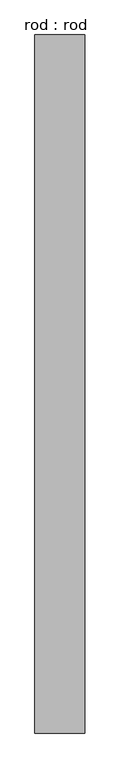
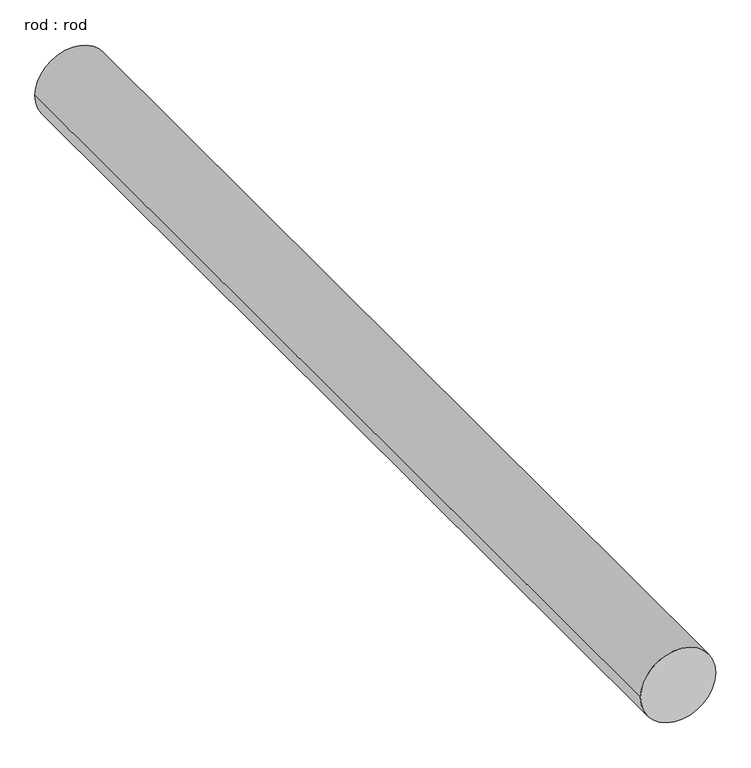
"""IFC4 building model written with IfcOpenShell, lengths in millimetres: proxy geometry, rod : rod."""

from ifc_helpers import new_model, si_unit, point, frame, frame_2d, origin, place, context, project, spatial, circle_curve, trimmed, segment, composite_curve, outline, extrude, source, transform, mapped, element, save


def rod_rod_a859c325(model_context):
    return source(origin(), model_context, "Body", "SweptSolid", [
        extrude(outline(composite_curve([segment(trimmed(circle_curve(frame_2d((0.0108462, 0.0)), 200.0), [point((0.0108462, 200.0))], [point((0.0108462, -200.0))], False, "CARTESIAN"), True, "CONTINUOUS"), segment(trimmed(circle_curve(frame_2d((0.0108462, 0.0)), 200.0), [point((0.0108462, -200.0))], [point((0.0108462, 200.0))], False, "CARTESIAN"), True, "CONTINUOUS")], self_intersect=False)), frame((0.0, 1304.1357802, 0.0), z_axis=(0.0, 1.0, 0.0), x_axis=(0.0, 0.0, 1.0)), (0.0, 0.0, 1.0), 5577.1856702),
    ])


if __name__ == "__main__":
    model = new_model("IFC4")
    model_context = context("Model", 3, world=origin())
    ifc_project = project(units=[si_unit("LENGTHUNIT", "METRE", prefix="MILLI")], contexts=[model_context])
    site = spatial("IfcSite", under=ifc_project)
    building = spatial("IfcBuilding", under=site)
    placement = place(None, origin())
    rod_rod_shape = rod_rod_a859c325(model_context)
    element("IfcBuildingElementProxy", 1, Name="rod : rod", ObjectType="rod : rod", at=placement, inside=building, context=model_context, shape_type="MappedRepresentation", body=[
        mapped(rod_rod_shape, transform((0.0, 0.0, 0.0), x_axis=(1.0, 0.0, 0.0), y_axis=(0.0, 1.0, 0.0), z_axis=(0.0, 0.0, 1.0))),
    ])
    save(model, "model.ifc")

# Revit data of these elements
# Type "rod : rod"
#   Default Elevation = 0
